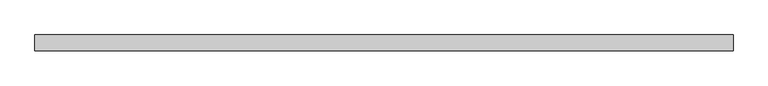
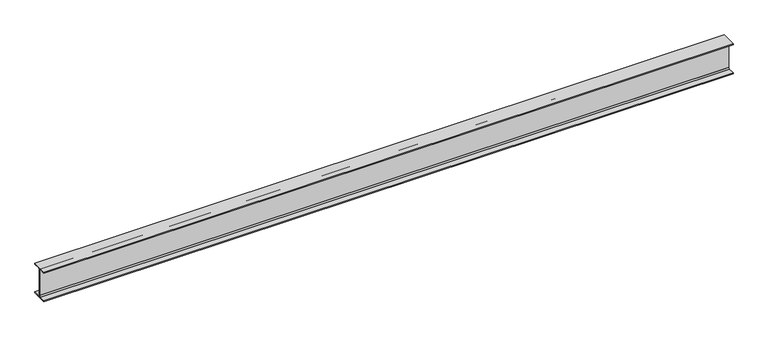
"""IFC4 building model written with IfcOpenShell, lengths in millimetres: beam geometry, 0912_Steel Framing_H-KSD3502 : H_SB_ASB_H-350x175x7x11."""

import ifcopenshell
import ifcopenshell.guid

model = None  # the IFC model being written
_history = None  # IfcOwnerHistory: only IFC2X3 demands one
_inside = {}  # id of a spatial element -> (the spatial element, [elements in it])
_under = {}  # id of a project, library or spatial element -> (it, [spatial elements below it])
_declared = {}  # id of a project -> (the project, [libraries it declares])
_typed = {}  # id of a type object -> (the type object, [elements of that type])
_made_of = {}  # id of a material, layer set ... -> (it, [elements and type objects made of it])


def new_model(schema):
    """Start an empty IFC model of exactly this schema.

    Asked for "IFC4X3", IfcOpenShell would pick the latest addendum, in which some entities
    have other attributes; the version numbers below select the first issue.
    IFC2X3 requires an IfcOwnerHistory on every rooted entity: one is made here for all.
    """
    global model, _history
    if schema == "IFC4X3":
        model = ifcopenshell.file(schema_version=(4, 3, 0, 0))
    else:
        model = ifcopenshell.file(schema=schema)
    _inside.clear()
    _under.clear()
    _declared.clear()
    _typed.clear()
    _made_of.clear()
    _history = None
    if model.schema == "IFC2X3":
        org = make("IfcOrganization", Name="unknown")
        user = make(
            "IfcPersonAndOrganization",
            ThePerson=make("IfcPerson", FamilyName="unknown"),
            TheOrganization=org,
        )
        app = make(
            "IfcApplication",
            ApplicationDeveloper=org,
            Version="unknown",
            ApplicationFullName="unknown",
            ApplicationIdentifier="unknown",
        )
        _history = make(
            "IfcOwnerHistory",
            OwningUser=user,
            OwningApplication=app,
            ChangeAction="ADDED",
            CreationDate=0,
        )
    return model


def make(cls, **values):
    """One entity of the class cls with the attributes given. An attribute that is None is left unset."""
    return model.create_entity(
        cls, **{name: value for name, value in values.items() if value is not None}
    )


def rooted(cls, **values):
    """An entity with a GlobalId (a new one), such as an element, a storey or a relation."""
    return make(cls, GlobalId=ifcopenshell.guid.new(), OwnerHistory=_history, **values)


def si_unit(unit_type, name, prefix=None):
    """IfcSIUnit, for example si_unit("LENGTHUNIT", "METRE", prefix="MILLI")."""
    return make("IfcSIUnit", UnitType=unit_type, Prefix=prefix, Name=name)


def assignment(units):
    """IfcUnitAssignment: the units of a project."""
    return None if units is None else make("IfcUnitAssignment", Units=units)


def point(xyz):
    """IfcCartesianPoint."""
    return None if xyz is None else make("IfcCartesianPoint", Coordinates=xyz)


def direction(xyz):
    """IfcDirection."""
    return None if xyz is None else make("IfcDirection", DirectionRatios=xyz)


def frame(location, z_axis=None, x_axis=None):
    """IfcAxis2Placement3D, a coordinate frame: its origin and axes. An axis left out is left unset."""
    return make(
        "IfcAxis2Placement3D",
        Location=point(location),
        Axis=direction(z_axis),
        RefDirection=direction(x_axis),
    )


def frame_2d(location, x_axis=None):
    """IfcAxis2Placement2D, a coordinate frame in the plane: its origin and x axis."""
    return make(
        "IfcAxis2Placement2D", Location=point(location), RefDirection=direction(x_axis)
    )


def origin():
    """The frame at (0, 0, 0) with its axes left unset."""
    return frame((0.0, 0.0, 0.0))


def place(relative_to, where):
    """IfcLocalPlacement: puts the frame where relative to a parent placement (None: the world)."""
    return make(
        "IfcLocalPlacement", PlacementRelTo=relative_to, RelativePlacement=where
    )


def context(
    kind, dimensions, precision=None, world=None, true_north=None, identifier=None
):
    """IfcGeometricRepresentationContext, for example the 3D "Model" context."""
    return make(
        "IfcGeometricRepresentationContext",
        ContextIdentifier=identifier,
        ContextType=kind,
        CoordinateSpaceDimension=dimensions,
        Precision=precision,
        WorldCoordinateSystem=world,
        TrueNorth=true_north,
    )


def project(units=None, contexts=None):
    """IfcProject with its units and contexts."""
    return rooted(
        "IfcProject",
        Name="project",
        RepresentationContexts=contexts,
        UnitsInContext=assignment(units),
    )


def spatial(cls, under=None, at=None, **own):
    """A site, building, storey or space (cls), placed at a placement, below another one or the project."""
    s = rooted(cls, ObjectPlacement=at, **own)
    if under is not None:
        _under.setdefault(under.id(), (under, []))[1].append(s)
    return s


def polyline(points):
    """IfcPolyline through the points."""
    return make("IfcPolyline", Points=[point(p) for p in points])


def circle_curve(where, radius):
    """IfcCircle in the frame where."""
    return make("IfcCircle", Position=where, Radius=radius)


def trimmed(basis, trim1, trim2, sense, master):
    """IfcTrimmedCurve: the piece of a basis curve between two trims."""
    return make(
        "IfcTrimmedCurve",
        BasisCurve=basis,
        Trim1=trim1,
        Trim2=trim2,
        SenseAgreement=sense,
        MasterRepresentation=master,
    )


def segment(curve, same_sense, transition):
    """IfcCompositeCurveSegment."""
    return make(
        "IfcCompositeCurveSegment",
        Transition=transition,
        SameSense=same_sense,
        ParentCurve=curve,
    )


def composite_curve(segments, self_intersect=None):
    """IfcCompositeCurve: segments joined end to end."""
    return make("IfcCompositeCurve", Segments=segments, SelfIntersect=self_intersect)


def outline(outer, holes=None, kind="AREA"):
    """IfcArbitraryClosedProfileDef: a profile drawn as a closed curve; with holes, ...WithVoids."""
    if holes is None:
        return make("IfcArbitraryClosedProfileDef", ProfileType=kind, OuterCurve=outer)
    return make(
        "IfcArbitraryProfileDefWithVoids",
        ProfileType=kind,
        OuterCurve=outer,
        InnerCurves=holes,
    )


def extrude(swept, where, along, depth):
    """IfcExtrudedAreaSolid: the profile swept, set in the frame where, extruded along a direction by depth."""
    return make(
        "IfcExtrudedAreaSolid",
        SweptArea=swept,
        Position=where,
        ExtrudedDirection=direction(along),
        Depth=depth,
    )


def shape(context_of_items, identifier, shape_type, items):
    """IfcShapeRepresentation: the items that make up one representation, for example the "Body"."""
    return make(
        "IfcShapeRepresentation",
        ContextOfItems=context_of_items,
        RepresentationIdentifier=identifier,
        RepresentationType=shape_type,
        Items=items,
    )


def source(mapping_origin, context_of_items, identifier, shape_type, items):
    """IfcRepresentationMap: a shape defined once, which mapped items show again and again."""
    return make(
        "IfcRepresentationMap",
        MappingOrigin=mapping_origin,
        MappedRepresentation=shape(context_of_items, identifier, shape_type, items),
    )


def transform(
    local_origin,
    x_axis=None,
    y_axis=None,
    z_axis=None,
    scale=None,
    scale2=None,
    scale3=None,
    uniform=True,
):
    """IfcCartesianTransformationOperator3D, or its non-uniform kind. x_axis, y_axis, z_axis: its Axis1, 2, 3."""
    if uniform:
        return make(
            "IfcCartesianTransformationOperator3D",
            Axis1=direction(x_axis),
            Axis2=direction(y_axis),
            LocalOrigin=point(local_origin),
            Scale=scale,
            Axis3=direction(z_axis),
        )
    return make(
        "IfcCartesianTransformationOperator3DnonUniform",
        Axis1=direction(x_axis),
        Axis2=direction(y_axis),
        LocalOrigin=point(local_origin),
        Scale=scale,
        Axis3=direction(z_axis),
        Scale2=scale2,
        Scale3=scale3,
    )


def mapped(mapping_source, mapping_target):
    """IfcMappedItem: shows the shape of a source again, moved by a transform."""
    return make(
        "IfcMappedItem", MappingSource=mapping_source, MappingTarget=mapping_target
    )


def made_of(thing, what):
    """Note that an element or type object is made of a material, layer set ...; save() writes the relation."""
    if what is not None:
        _made_of.setdefault(what.id(), (what, []))[1].append(thing)
    return thing


def element(
    cls,
    number,
    at=None,
    inside=None,
    cuts=None,
    type_object=None,
    material=None,
    context=None,
    identifier="Body",
    shape_type=None,
    held_by="IfcProductDefinitionShape",
    body=None,
    shapes=None,
    **own,
):
    """One element of the class cls, such as IfcWall. Its Tag is "e" and its number.

    at: its placement. inside: the storey or other place that contains it. cuts: it is an
    opening in that element (IfcRelVoidsElement). A single representation is given by context,
    identifier, shape_type and body (its items); several are given by shapes. held_by: the class
    of the entity that holds the representations. save() writes the other relations.
    """
    e = rooted(cls, Tag="e%d" % number, ObjectPlacement=at, **own)
    if body is not None:
        shapes = [shape(context, identifier, shape_type, body)]
    if shapes is not None:
        e.Representation = make(held_by, Representations=shapes)
    if inside is not None:
        _inside.setdefault(inside.id(), (inside, []))[1].append(e)
    if cuts is not None:
        rooted(
            "IfcRelVoidsElement", RelatingBuildingElement=cuts, RelatedOpeningElement=e
        )
    if type_object is not None:
        _typed.setdefault(type_object.id(), (type_object, []))[1].append(e)
    return made_of(e, material)


def aggregate(whole, parts):
    """IfcRelAggregates: a whole, such as a stair, and the parts it consists of."""
    return rooted("IfcRelAggregates", RelatingObject=whole, RelatedObjects=parts)


def save(model, path):
    """Write the relations noted so far, then the file.

    IfcRelAggregates (storeys below a building ...), IfcRelContainedInSpatialStructure (elements
    in a storey), IfcRelDefinesByType, IfcRelAssociatesMaterial and IfcRelDeclares: one each for
    every whole, place, type object, material and project.
    """
    for whole, parts in _under.values():
        aggregate(whole, parts)
    for where, things in _inside.values():
        rooted(
            "IfcRelContainedInSpatialStructure",
            RelatedElements=things,
            RelatingStructure=where,
        )
    for kind, things in _typed.values():
        rooted("IfcRelDefinesByType", RelatedObjects=things, RelatingType=kind)
    for what, things in _made_of.values():
        rooted("IfcRelAssociatesMaterial", RelatedObjects=things, RelatingMaterial=what)
    for by, libraries in _declared.values():
        rooted("IfcRelDeclares", RelatingContext=by, RelatedDefinitions=libraries)
    model.write(path)


def beam_a6d55a04(model_context):
    return source(origin(), model_context, "Body", "SweptSolid", [
        extrude(outline(composite_curve([segment(polyline([(87.5, -164.0), (87.5, -175.0), (-87.5, -175.0), (-87.5, -164.0), (-17.5, -164.0)]), True, "CONTINUOUS"), segment(trimmed(circle_curve(frame_2d((-17.5, -150.0)), 14.0), [point((-17.5, -164.0))], [point((-3.5, -150.0))], True, "CARTESIAN"), True, "CONTINUOUS"), segment(polyline([(-3.5, -150.0), (-3.5, 150.0)]), True, "CONTINUOUS"), segment(trimmed(circle_curve(frame_2d((-17.5, 150.0)), 14.0), [point((-3.5, 150.0))], [point((-17.5, 164.0))], True, "CARTESIAN"), True, "CONTINUOUS"), segment(polyline([(-17.5, 164.0), (-87.5, 164.0), (-87.5, 175.0), (87.5, 175.0), (87.5, 164.0), (17.5, 164.0)]), True, "CONTINUOUS"), segment(trimmed(circle_curve(frame_2d((17.5, 150.0)), 14.0), [point((17.5, 164.0))], [point((3.5, 150.0))], True, "CARTESIAN"), True, "CONTINUOUS"), segment(polyline([(3.5, 150.0), (3.5, -150.0)]), True, "CONTINUOUS"), segment(trimmed(circle_curve(frame_2d((17.5, -150.0)), 14.0), [point((3.5, -150.0))], [point((17.5, -164.0))], True, "CARTESIAN"), True, "CONTINUOUS"), segment(polyline([(17.5, -164.0), (87.5, -164.0)]), True, "CONTINUOUS")], self_intersect=False)), frame((-3837.3, 0.0, 0.0), z_axis=(1.0, 0.0, 0.0), x_axis=(0.0, 1.0, 0.0)), (0.0, 0.0, 1.0), 7674.6),
    ])


if __name__ == "__main__":
    model = new_model("IFC4")
    model_context = context("Model", 3, world=origin())
    ifc_project = project(units=[si_unit("LENGTHUNIT", "METRE", prefix="MILLI")], contexts=[model_context])
    site = spatial("IfcSite", under=ifc_project)
    building = spatial("IfcBuilding", under=site)
    placement = place(None, origin())
    beam_shape = beam_a6d55a04(model_context)
    element("IfcBeam", 1, ObjectType="0912_Steel Framing_H-KSD3502 : H_SB_ASB_H-350x175x7x11", at=placement, inside=building, context=model_context, shape_type="MappedRepresentation", body=[
        mapped(beam_shape, transform((0.0, 0.0, 0.0), x_axis=(1.0, 0.0, 0.0), y_axis=(0.0, 1.0, 0.0), z_axis=(0.0, 0.0, 1.0))),
    ])
    save(model, "model.ifc")

# Revit data of these elements
# Type "0912_Steel Framing_H-KSD3502 : H_SB_ASB_H-350x175x7x11"
#   H_WM Code_1 = "S01AA002-00001 | Main Steel Structure Fabrication Work | Shelter/Building | Medium Steel - Standard (90KG/M>Weight≥30KG/M) | Material: (   )"
#   H_WM Code_2 = "S03AA028-00001 | Main Steel Structure Erection Work | Shelter/Building | Medium Steel (90KG/M>Weight≥30KG/M) | Material: (   )"
#   H_WM Code_3 = "S01AA010-00001 | Main Steel Structure Fabrication Work | Shelter/Building | Steel Painting/Coating | for Non-Fireproofed Steel Surface, Surface Preparation, Primer, Second & Final Coat | Material: (   )"
#   H_Q'ty Cal Type Tag = "SB-Q2"
#   Width = 17.5 cm
#   Web Thickness = 0.7 cm
#   Web Fillet = 1.4 cm
#   Warping Constant = 282000.0 cm⁶
#   W = 0
#   Torsional Moment of Inertia = 19.4042 cm⁴
#   Section Area = 63.14 cm²
#   Plastic Modulus weak axis = 174.0 cm³
#   Plastic Modulus strong axis = 868.0 cm³
#   Perimeter = 1.36 m²/m
#   Nominal Weight = 49.60 kgf/m
#   Moment of Inertia weak axis = 984.00 cm⁴
#   Moment of Inertia strong axis = 13600.00 cm⁴
#   Height = 35.0 cm
#   Flange Thickness = 1.1 cm
#   Elastic Modulus weak axis = 112.0 cm³
#   Elastic Modulus strong axis = 775.0 cm³
#   Centroid Vertical = 17.5 cm
#   Centroid Horizontal = 8.75 cm
#   Ix = 136000000
#   Length [instance default] = 1.5240 m
#   Zx = 868000
#   b = 0.1750 m
#   h = 0.3500 m
#   r = 0.0140 m
#   s = 0.0070 m
#   t = 0.0110 m
#   A = 0.006314 m²
#   Structural Material [instance default] = Steel, 45-345
#   Assembly Code = ""
# Element 1 (IfcBeam, "0912_Steel Framing_H-KSD3502 : H_SB_ASB_H-350x175x7x11")
#   Structural Material = none
# Materials
#   "Steel, 45-345": class "Metal", colour RGB 189 187 185, transparency 0, Description = "Steel 345 MPa", Cost = 0
